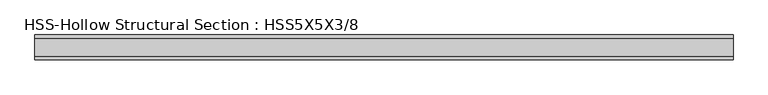
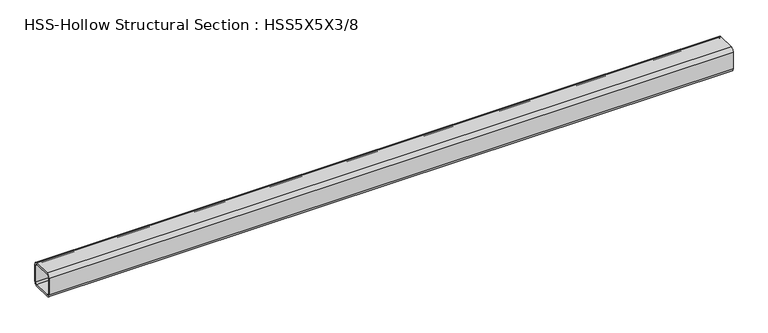
"""IFC4 building model written with IfcOpenShell, lengths in millimetres: member geometry, HSS-Hollow Structural Section : HSS5X5X3/8."""

from ifc_helpers import new_model, si_unit, point, frame, frame_2d, origin, place, context, project, spatial, polyline, circle_curve, trimmed, segment, composite_curve, outline, extrude, source, transform, mapped, element, save


def hss_hollow_structural_section_hss5x5x3_8_2df68ff6(model_context):
    return source(origin(), model_context, "Body", "SweptSolid", [
        extrude(outline(composite_curve([segment(polyline([(63.5, 45.7708), (63.5, -45.7708)]), True, "CONTINUOUS"), segment(trimmed(circle_curve(frame_2d((45.7708, -45.7708)), 17.7292), [point((63.5, -45.7708))], [point((45.7708, -63.5))], False, "CARTESIAN"), True, "CONTINUOUS"), segment(polyline([(45.7708, -63.5), (-45.7708, -63.5)]), True, "CONTINUOUS"), segment(trimmed(circle_curve(frame_2d((-45.7708, -45.7708)), 17.7292), [point((-45.7708, -63.5))], [point((-63.5, -45.7708))], False, "CARTESIAN"), True, "CONTINUOUS"), segment(polyline([(-63.5, -45.7708), (-63.5, 45.7708)]), True, "CONTINUOUS"), segment(trimmed(circle_curve(frame_2d((-45.7708, 45.7708)), 17.7292), [point((-63.5, 45.7708))], [point((-45.7708, 63.5))], False, "CARTESIAN"), True, "CONTINUOUS"), segment(polyline([(-45.7708, 63.5), (45.7708, 63.5)]), True, "CONTINUOUS"), segment(trimmed(circle_curve(frame_2d((45.7708, 45.7708)), 17.7292), [point((45.7708, 63.5))], [point((63.5, 45.7708))], False, "CARTESIAN"), True, "CONTINUOUS")], self_intersect=False), holes=[composite_curve([segment(trimmed(circle_curve(frame_2d((-45.7708, 45.7708)), 8.8646), [point((-45.7708, 54.6354))], [point((-54.6354, 45.7708))], True, "CARTESIAN"), True, "CONTINUOUS"), segment(polyline([(-54.6354, 45.7708), (-54.6354, -45.7708)]), True, "CONTINUOUS"), segment(trimmed(circle_curve(frame_2d((-45.7708, -45.7708)), 8.8646), [point((-54.6354, -45.7708))], [point((-45.7708, -54.6354))], True, "CARTESIAN"), True, "CONTINUOUS"), segment(polyline([(-45.7708, -54.6354), (45.7708, -54.6354)]), True, "CONTINUOUS"), segment(trimmed(circle_curve(frame_2d((45.7708, -45.7708)), 8.8646), [point((45.7708, -54.6354))], [point((54.6354, -45.7708))], True, "CARTESIAN"), True, "CONTINUOUS"), segment(polyline([(54.6354, -45.7708), (54.6354, 45.7708)]), True, "CONTINUOUS"), segment(trimmed(circle_curve(frame_2d((45.7708, 45.7708)), 8.8646), [point((54.6354, 45.7708))], [point((45.7708, 54.6354))], True, "CARTESIAN"), True, "CONTINUOUS"), segment(polyline([(45.7708, 54.6354), (-45.7708, 54.6354)]), True, "CONTINUOUS")], self_intersect=False)]), frame((-1778.3838811, 0.0, 0.0), z_axis=(1.0, 0.0, 0.0), x_axis=(0.0, 1.0, 0.0)), (0.0, 0.0, 1.0), 3556.7677621),
    ])


if __name__ == "__main__":
    model = new_model("IFC4")
    model_context = context("Model", 3, world=origin())
    ifc_project = project(units=[si_unit("LENGTHUNIT", "METRE", prefix="MILLI")], contexts=[model_context])
    site = spatial("IfcSite", under=ifc_project)
    building = spatial("IfcBuilding", under=site)
    placement = place(None, origin())
    hss_hollow_structural_section_hss5x5x3_8_shape = hss_hollow_structural_section_hss5x5x3_8_2df68ff6(model_context)
    element("IfcMember", 1, ObjectType="HSS-Hollow Structural Section : HSS5X5X3/8", at=placement, inside=building, context=model_context, shape_type="MappedRepresentation", body=[
        mapped(hss_hollow_structural_section_hss5x5x3_8_shape, transform((0.0, 0.0, 0.0), x_axis=(1.0, 0.0, 0.0), y_axis=(0.0, 1.0, 0.0), z_axis=(0.0, 0.0, 1.0))),
    ])
    save(model, "model.ifc")

# Revit data of these elements
# Type "HSS-Hollow Structural Section : HSS5X5X3/8"
#   Assembly Code = "B10"
#   Shape = "Square"
#   W = 22.3
#   Ht = 0' - 5"
#   Length [instance default] = 5' - 0"
#   b = 0' - 5"
#   kr = 0' - 0.698"
#   t = 0' - 0.349"
#   A = 0.0429167 SF
#   Structural Material [instance default] = Steel ASTM A500, Grade B, Rectangular and Square
# Element 1 (IfcMember, "HSS-Hollow Structural Section : HSS5X5X3/8")
#   Materials on its faces: "Steel ASTM A500, Grade B, Rectangular and Square"
# Materials
#   "Steel ASTM A500, Grade B, Rectangular and Square": class "Metal", colour RGB 199 199 199, transparency 0, Description = "Carbon steel", Cost = 0
